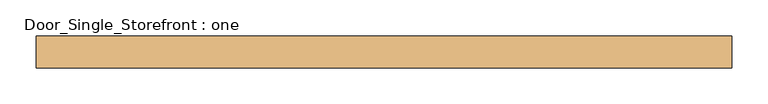
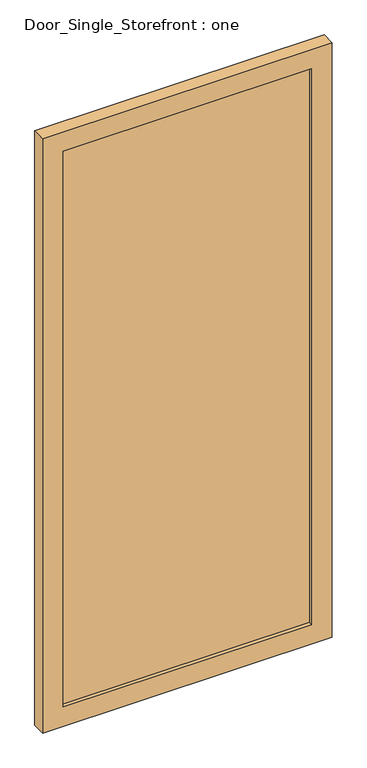
"""IFC4 building model written with IfcOpenShell, lengths in millimetres: door geometry, Door_Single_Storefront : one."""

import ifcopenshell
import ifcopenshell.guid

model = None  # the IFC model being written
_history = None  # IfcOwnerHistory: only IFC2X3 demands one
_inside = {}  # id of a spatial element -> (the spatial element, [elements in it])
_under = {}  # id of a project, library or spatial element -> (it, [spatial elements below it])
_declared = {}  # id of a project -> (the project, [libraries it declares])
_typed = {}  # id of a type object -> (the type object, [elements of that type])
_made_of = {}  # id of a material, layer set ... -> (it, [elements and type objects made of it])


def new_model(schema):
    """Start an empty IFC model of exactly this schema.

    Asked for "IFC4X3", IfcOpenShell would pick the latest addendum, in which some entities
    have other attributes; the version numbers below select the first issue.
    IFC2X3 requires an IfcOwnerHistory on every rooted entity: one is made here for all.
    """
    global model, _history
    if schema == "IFC4X3":
        model = ifcopenshell.file(schema_version=(4, 3, 0, 0))
    else:
        model = ifcopenshell.file(schema=schema)
    _inside.clear()
    _under.clear()
    _declared.clear()
    _typed.clear()
    _made_of.clear()
    _history = None
    if model.schema == "IFC2X3":
        org = make("IfcOrganization", Name="unknown")
        user = make(
            "IfcPersonAndOrganization",
            ThePerson=make("IfcPerson", FamilyName="unknown"),
            TheOrganization=org,
        )
        app = make(
            "IfcApplication",
            ApplicationDeveloper=org,
            Version="unknown",
            ApplicationFullName="unknown",
            ApplicationIdentifier="unknown",
        )
        _history = make(
            "IfcOwnerHistory",
            OwningUser=user,
            OwningApplication=app,
            ChangeAction="ADDED",
            CreationDate=0,
        )
    return model


def make(cls, **values):
    """One entity of the class cls with the attributes given. An attribute that is None is left unset."""
    return model.create_entity(
        cls, **{name: value for name, value in values.items() if value is not None}
    )


def rooted(cls, **values):
    """An entity with a GlobalId (a new one), such as an element, a storey or a relation."""
    return make(cls, GlobalId=ifcopenshell.guid.new(), OwnerHistory=_history, **values)


def si_unit(unit_type, name, prefix=None):
    """IfcSIUnit, for example si_unit("LENGTHUNIT", "METRE", prefix="MILLI")."""
    return make("IfcSIUnit", UnitType=unit_type, Prefix=prefix, Name=name)


def assignment(units):
    """IfcUnitAssignment: the units of a project."""
    return None if units is None else make("IfcUnitAssignment", Units=units)


def point(xyz):
    """IfcCartesianPoint."""
    return None if xyz is None else make("IfcCartesianPoint", Coordinates=xyz)


def direction(xyz):
    """IfcDirection."""
    return None if xyz is None else make("IfcDirection", DirectionRatios=xyz)


def frame(location, z_axis=None, x_axis=None):
    """IfcAxis2Placement3D, a coordinate frame: its origin and axes. An axis left out is left unset."""
    return make(
        "IfcAxis2Placement3D",
        Location=point(location),
        Axis=direction(z_axis),
        RefDirection=direction(x_axis),
    )


def origin():
    """The frame at (0, 0, 0) with its axes left unset."""
    return frame((0.0, 0.0, 0.0))


def place(relative_to, where):
    """IfcLocalPlacement: puts the frame where relative to a parent placement (None: the world)."""
    return make(
        "IfcLocalPlacement", PlacementRelTo=relative_to, RelativePlacement=where
    )


def context(
    kind, dimensions, precision=None, world=None, true_north=None, identifier=None
):
    """IfcGeometricRepresentationContext, for example the 3D "Model" context."""
    return make(
        "IfcGeometricRepresentationContext",
        ContextIdentifier=identifier,
        ContextType=kind,
        CoordinateSpaceDimension=dimensions,
        Precision=precision,
        WorldCoordinateSystem=world,
        TrueNorth=true_north,
    )


def project(units=None, contexts=None):
    """IfcProject with its units and contexts."""
    return rooted(
        "IfcProject",
        Name="project",
        RepresentationContexts=contexts,
        UnitsInContext=assignment(units),
    )


def spatial(cls, under=None, at=None, **own):
    """A site, building, storey or space (cls), placed at a placement, below another one or the project."""
    s = rooted(cls, ObjectPlacement=at, **own)
    if under is not None:
        _under.setdefault(under.id(), (under, []))[1].append(s)
    return s


def polyline(points):
    """IfcPolyline through the points."""
    return make("IfcPolyline", Points=[point(p) for p in points])


def outline(outer, holes=None, kind="AREA"):
    """IfcArbitraryClosedProfileDef: a profile drawn as a closed curve; with holes, ...WithVoids."""
    if holes is None:
        return make("IfcArbitraryClosedProfileDef", ProfileType=kind, OuterCurve=outer)
    return make(
        "IfcArbitraryProfileDefWithVoids",
        ProfileType=kind,
        OuterCurve=outer,
        InnerCurves=holes,
    )


def extrude(swept, where, along, depth):
    """IfcExtrudedAreaSolid: the profile swept, set in the frame where, extruded along a direction by depth."""
    return make(
        "IfcExtrudedAreaSolid",
        SweptArea=swept,
        Position=where,
        ExtrudedDirection=direction(along),
        Depth=depth,
    )


def shape(context_of_items, identifier, shape_type, items):
    """IfcShapeRepresentation: the items that make up one representation, for example the "Body"."""
    return make(
        "IfcShapeRepresentation",
        ContextOfItems=context_of_items,
        RepresentationIdentifier=identifier,
        RepresentationType=shape_type,
        Items=items,
    )


def source(mapping_origin, context_of_items, identifier, shape_type, items):
    """IfcRepresentationMap: a shape defined once, which mapped items show again and again."""
    return make(
        "IfcRepresentationMap",
        MappingOrigin=mapping_origin,
        MappedRepresentation=shape(context_of_items, identifier, shape_type, items),
    )


def transform(
    local_origin,
    x_axis=None,
    y_axis=None,
    z_axis=None,
    scale=None,
    scale2=None,
    scale3=None,
    uniform=True,
):
    """IfcCartesianTransformationOperator3D, or its non-uniform kind. x_axis, y_axis, z_axis: its Axis1, 2, 3."""
    if uniform:
        return make(
            "IfcCartesianTransformationOperator3D",
            Axis1=direction(x_axis),
            Axis2=direction(y_axis),
            LocalOrigin=point(local_origin),
            Scale=scale,
            Axis3=direction(z_axis),
        )
    return make(
        "IfcCartesianTransformationOperator3DnonUniform",
        Axis1=direction(x_axis),
        Axis2=direction(y_axis),
        LocalOrigin=point(local_origin),
        Scale=scale,
        Axis3=direction(z_axis),
        Scale2=scale2,
        Scale3=scale3,
    )


def mapped(mapping_source, mapping_target):
    """IfcMappedItem: shows the shape of a source again, moved by a transform."""
    return make(
        "IfcMappedItem", MappingSource=mapping_source, MappingTarget=mapping_target
    )


def made_of(thing, what):
    """Note that an element or type object is made of a material, layer set ...; save() writes the relation."""
    if what is not None:
        _made_of.setdefault(what.id(), (what, []))[1].append(thing)
    return thing


def element(
    cls,
    number,
    at=None,
    inside=None,
    cuts=None,
    type_object=None,
    material=None,
    context=None,
    identifier="Body",
    shape_type=None,
    held_by="IfcProductDefinitionShape",
    body=None,
    shapes=None,
    **own,
):
    """One element of the class cls, such as IfcWall. Its Tag is "e" and its number.

    at: its placement. inside: the storey or other place that contains it. cuts: it is an
    opening in that element (IfcRelVoidsElement). A single representation is given by context,
    identifier, shape_type and body (its items); several are given by shapes. held_by: the class
    of the entity that holds the representations. save() writes the other relations.
    """
    e = rooted(cls, Tag="e%d" % number, ObjectPlacement=at, **own)
    if body is not None:
        shapes = [shape(context, identifier, shape_type, body)]
    if shapes is not None:
        e.Representation = make(held_by, Representations=shapes)
    if inside is not None:
        _inside.setdefault(inside.id(), (inside, []))[1].append(e)
    if cuts is not None:
        rooted(
            "IfcRelVoidsElement", RelatingBuildingElement=cuts, RelatedOpeningElement=e
        )
    if type_object is not None:
        _typed.setdefault(type_object.id(), (type_object, []))[1].append(e)
    return made_of(e, material)


def aggregate(whole, parts):
    """IfcRelAggregates: a whole, such as a stair, and the parts it consists of."""
    return rooted("IfcRelAggregates", RelatingObject=whole, RelatedObjects=parts)


def save(model, path):
    """Write the relations noted so far, then the file.

    IfcRelAggregates (storeys below a building ...), IfcRelContainedInSpatialStructure (elements
    in a storey), IfcRelDefinesByType, IfcRelAssociatesMaterial and IfcRelDeclares: one each for
    every whole, place, type object, material and project.
    """
    for whole, parts in _under.values():
        aggregate(whole, parts)
    for where, things in _inside.values():
        rooted(
            "IfcRelContainedInSpatialStructure",
            RelatedElements=things,
            RelatingStructure=where,
        )
    for kind, things in _typed.values():
        rooted("IfcRelDefinesByType", RelatedObjects=things, RelatingType=kind)
    for what, things in _made_of.values():
        rooted("IfcRelAssociatesMaterial", RelatedObjects=things, RelatingMaterial=what)
    for by, libraries in _declared.values():
        rooted("IfcRelDeclares", RelatingContext=by, RelatedDefinitions=libraries)
    model.write(path)


def door_single_storefront_one_c6851394(model_context):
    return source(origin(), model_context, "Body", "SweptSolid", [
        extrude(outline(polyline([(414.734375, -6.35), (-414.734375, -6.35), (-414.734375, 12.7), (414.734375, 12.7), (414.734375, -6.35)])), frame((0.0, 0.0, 68.2625), z_axis=(0.0, 0.0, 1.0), x_axis=(1.0, 0.0, 0.0)), (0.0, 0.0, 1.0), 1958.975),
        extrude(outline(polyline([(2095.5, -482.996875), (0.0, -482.996875), (0.0, 482.996875), (2095.5, 482.996875), (2095.5, -482.996875)]), holes=[polyline([(68.2625, 414.734375), (68.2625, -414.734375), (2027.2375, -414.734375), (2027.2375, 414.734375), (68.2625, 414.734375)])]), frame((0.0, -19.05, 0.0), z_axis=(0.0, 1.0, 0.0), x_axis=(0.0, 0.0, 1.0)), (0.0, 0.0, 1.0), 44.45),
    ])


if __name__ == "__main__":
    model = new_model("IFC4")
    model_context = context("Model", 3, world=origin())
    ifc_project = project(units=[si_unit("LENGTHUNIT", "METRE", prefix="MILLI")], contexts=[model_context])
    site = spatial("IfcSite", under=ifc_project)
    building = spatial("IfcBuilding", under=site)
    placement = place(None, origin())
    door_single_storefront_one_shape = door_single_storefront_one_c6851394(model_context)
    element("IfcDoor", 1, ObjectType="Door_Single_Storefront : one", at=placement, inside=building, context=model_context, shape_type="MappedRepresentation", body=[
        mapped(door_single_storefront_one_shape, transform((0.0, 0.0, 0.0), x_axis=(1.0, 0.0, 0.0), y_axis=(0.0, 1.0, 0.0), z_axis=(0.0, 0.0, 1.0))),
    ])
    save(model, "model.ifc")

# Revit data of these elements
# Type "Door_Single_Storefront : one"
#   Type Mark = "29"
#   OD_DS_Door_Material = "ALUM./GLAZING"
#   OD_DS_Door_Type = "STOREFRONT (NARROW STILE)"
#   OD_DS_Lockset = "ENTRY LOCK (INSIDE ADA LEVER ALWAYS ACTIVE)"
#   Analytic Construction = "<None>"
#   angle open [instance default] = 132.952°
#   Stile_Width = 0' - 2 11/16"
#   Door_Thickness = 0' - 1 3/4"
#   Door_Offset = 0' - 1"
#   Glass_Material = TEMPERED INSULATED GLAZING (CARDINAL GLASS LoĒ²-240\nOR EQUIVALENT)
#   Frame_Material = KAWNEER 260 INSULCLADTM THERMAL ENTRANCE - CLEAR ANODIZED ALUM.
#   Function = (empty or 0)
# Element 1 (IfcDoor, "Door_Single_Storefront : one")
#   angle open = 170.00°
#   Materials on its faces: "KAWNEER 260 INSULCLADTM THERMAL ENTRANCE - CLEAR ANODIZED ALUM.", "TEMPERED INSULATED GLAZING (CARDINAL GLASS LoĒ²-240\nOR EQUIVALENT)"
# Materials
#   "TEMPERED INSULATED GLAZING (CARDINAL GLASS LoĒ²-240\nOR EQUIVALENT)": class "Glass", colour RGB 196 205 210, transparency 0.85, Description = "Soda Lime Glass", Cost = 0
#   "KAWNEER 260 INSULCLADTM THERMAL ENTRANCE - CLEAR ANODIZED ALUM.": class "Metal", colour RGB 244 244 244, transparency 0, Description = "Aluminum 6061", Cost = 0
